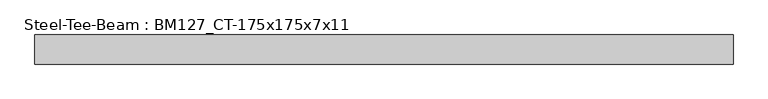
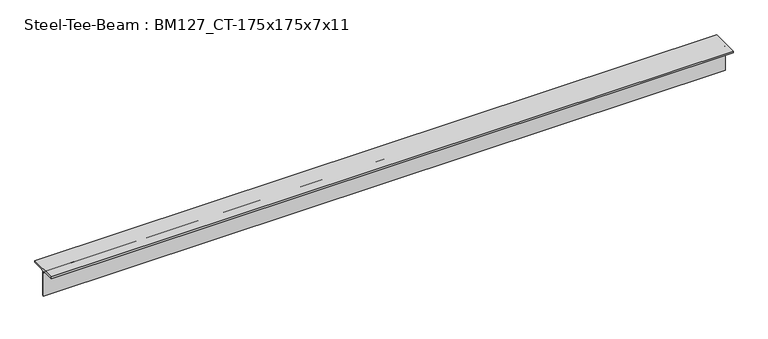
"""IFC4 building model written with IfcOpenShell, lengths in millimetres: beam geometry, Steel-Tee-Beam : BM127_CT-175x175x7x11."""

import ifcopenshell
import ifcopenshell.guid

model = None  # the IFC model being written
_history = None  # IfcOwnerHistory: only IFC2X3 demands one
_inside = {}  # id of a spatial element -> (the spatial element, [elements in it])
_under = {}  # id of a project, library or spatial element -> (it, [spatial elements below it])
_declared = {}  # id of a project -> (the project, [libraries it declares])
_typed = {}  # id of a type object -> (the type object, [elements of that type])
_made_of = {}  # id of a material, layer set ... -> (it, [elements and type objects made of it])


def new_model(schema):
    """Start an empty IFC model of exactly this schema.

    Asked for "IFC4X3", IfcOpenShell would pick the latest addendum, in which some entities
    have other attributes; the version numbers below select the first issue.
    IFC2X3 requires an IfcOwnerHistory on every rooted entity: one is made here for all.
    """
    global model, _history
    if schema == "IFC4X3":
        model = ifcopenshell.file(schema_version=(4, 3, 0, 0))
    else:
        model = ifcopenshell.file(schema=schema)
    _inside.clear()
    _under.clear()
    _declared.clear()
    _typed.clear()
    _made_of.clear()
    _history = None
    if model.schema == "IFC2X3":
        org = make("IfcOrganization", Name="unknown")
        user = make(
            "IfcPersonAndOrganization",
            ThePerson=make("IfcPerson", FamilyName="unknown"),
            TheOrganization=org,
        )
        app = make(
            "IfcApplication",
            ApplicationDeveloper=org,
            Version="unknown",
            ApplicationFullName="unknown",
            ApplicationIdentifier="unknown",
        )
        _history = make(
            "IfcOwnerHistory",
            OwningUser=user,
            OwningApplication=app,
            ChangeAction="ADDED",
            CreationDate=0,
        )
    return model


def make(cls, **values):
    """One entity of the class cls with the attributes given. An attribute that is None is left unset."""
    return model.create_entity(
        cls, **{name: value for name, value in values.items() if value is not None}
    )


def rooted(cls, **values):
    """An entity with a GlobalId (a new one), such as an element, a storey or a relation."""
    return make(cls, GlobalId=ifcopenshell.guid.new(), OwnerHistory=_history, **values)


def si_unit(unit_type, name, prefix=None):
    """IfcSIUnit, for example si_unit("LENGTHUNIT", "METRE", prefix="MILLI")."""
    return make("IfcSIUnit", UnitType=unit_type, Prefix=prefix, Name=name)


def assignment(units):
    """IfcUnitAssignment: the units of a project."""
    return None if units is None else make("IfcUnitAssignment", Units=units)


def point(xyz):
    """IfcCartesianPoint."""
    return None if xyz is None else make("IfcCartesianPoint", Coordinates=xyz)


def direction(xyz):
    """IfcDirection."""
    return None if xyz is None else make("IfcDirection", DirectionRatios=xyz)


def frame(location, z_axis=None, x_axis=None):
    """IfcAxis2Placement3D, a coordinate frame: its origin and axes. An axis left out is left unset."""
    return make(
        "IfcAxis2Placement3D",
        Location=point(location),
        Axis=direction(z_axis),
        RefDirection=direction(x_axis),
    )


def frame_2d(location, x_axis=None):
    """IfcAxis2Placement2D, a coordinate frame in the plane: its origin and x axis."""
    return make(
        "IfcAxis2Placement2D", Location=point(location), RefDirection=direction(x_axis)
    )


def origin():
    """The frame at (0, 0, 0) with its axes left unset."""
    return frame((0.0, 0.0, 0.0))


def place(relative_to, where):
    """IfcLocalPlacement: puts the frame where relative to a parent placement (None: the world)."""
    return make(
        "IfcLocalPlacement", PlacementRelTo=relative_to, RelativePlacement=where
    )


def context(
    kind, dimensions, precision=None, world=None, true_north=None, identifier=None
):
    """IfcGeometricRepresentationContext, for example the 3D "Model" context."""
    return make(
        "IfcGeometricRepresentationContext",
        ContextIdentifier=identifier,
        ContextType=kind,
        CoordinateSpaceDimension=dimensions,
        Precision=precision,
        WorldCoordinateSystem=world,
        TrueNorth=true_north,
    )


def project(units=None, contexts=None):
    """IfcProject with its units and contexts."""
    return rooted(
        "IfcProject",
        Name="project",
        RepresentationContexts=contexts,
        UnitsInContext=assignment(units),
    )


def spatial(cls, under=None, at=None, **own):
    """A site, building, storey or space (cls), placed at a placement, below another one or the project."""
    s = rooted(cls, ObjectPlacement=at, **own)
    if under is not None:
        _under.setdefault(under.id(), (under, []))[1].append(s)
    return s


def polyline(points):
    """IfcPolyline through the points."""
    return make("IfcPolyline", Points=[point(p) for p in points])


def circle_curve(where, radius):
    """IfcCircle in the frame where."""
    return make("IfcCircle", Position=where, Radius=radius)


def trimmed(basis, trim1, trim2, sense, master):
    """IfcTrimmedCurve: the piece of a basis curve between two trims."""
    return make(
        "IfcTrimmedCurve",
        BasisCurve=basis,
        Trim1=trim1,
        Trim2=trim2,
        SenseAgreement=sense,
        MasterRepresentation=master,
    )


def segment(curve, same_sense, transition):
    """IfcCompositeCurveSegment."""
    return make(
        "IfcCompositeCurveSegment",
        Transition=transition,
        SameSense=same_sense,
        ParentCurve=curve,
    )


def composite_curve(segments, self_intersect=None):
    """IfcCompositeCurve: segments joined end to end."""
    return make("IfcCompositeCurve", Segments=segments, SelfIntersect=self_intersect)


def outline(outer, holes=None, kind="AREA"):
    """IfcArbitraryClosedProfileDef: a profile drawn as a closed curve; with holes, ...WithVoids."""
    if holes is None:
        return make("IfcArbitraryClosedProfileDef", ProfileType=kind, OuterCurve=outer)
    return make(
        "IfcArbitraryProfileDefWithVoids",
        ProfileType=kind,
        OuterCurve=outer,
        InnerCurves=holes,
    )


def extrude(swept, where, along, depth):
    """IfcExtrudedAreaSolid: the profile swept, set in the frame where, extruded along a direction by depth."""
    return make(
        "IfcExtrudedAreaSolid",
        SweptArea=swept,
        Position=where,
        ExtrudedDirection=direction(along),
        Depth=depth,
    )


def shape(context_of_items, identifier, shape_type, items):
    """IfcShapeRepresentation: the items that make up one representation, for example the "Body"."""
    return make(
        "IfcShapeRepresentation",
        ContextOfItems=context_of_items,
        RepresentationIdentifier=identifier,
        RepresentationType=shape_type,
        Items=items,
    )


def source(mapping_origin, context_of_items, identifier, shape_type, items):
    """IfcRepresentationMap: a shape defined once, which mapped items show again and again."""
    return make(
        "IfcRepresentationMap",
        MappingOrigin=mapping_origin,
        MappedRepresentation=shape(context_of_items, identifier, shape_type, items),
    )


def transform(
    local_origin,
    x_axis=None,
    y_axis=None,
    z_axis=None,
    scale=None,
    scale2=None,
    scale3=None,
    uniform=True,
):
    """IfcCartesianTransformationOperator3D, or its non-uniform kind. x_axis, y_axis, z_axis: its Axis1, 2, 3."""
    if uniform:
        return make(
            "IfcCartesianTransformationOperator3D",
            Axis1=direction(x_axis),
            Axis2=direction(y_axis),
            LocalOrigin=point(local_origin),
            Scale=scale,
            Axis3=direction(z_axis),
        )
    return make(
        "IfcCartesianTransformationOperator3DnonUniform",
        Axis1=direction(x_axis),
        Axis2=direction(y_axis),
        LocalOrigin=point(local_origin),
        Scale=scale,
        Axis3=direction(z_axis),
        Scale2=scale2,
        Scale3=scale3,
    )


def mapped(mapping_source, mapping_target):
    """IfcMappedItem: shows the shape of a source again, moved by a transform."""
    return make(
        "IfcMappedItem", MappingSource=mapping_source, MappingTarget=mapping_target
    )


def made_of(thing, what):
    """Note that an element or type object is made of a material, layer set ...; save() writes the relation."""
    if what is not None:
        _made_of.setdefault(what.id(), (what, []))[1].append(thing)
    return thing


def element(
    cls,
    number,
    at=None,
    inside=None,
    cuts=None,
    type_object=None,
    material=None,
    context=None,
    identifier="Body",
    shape_type=None,
    held_by="IfcProductDefinitionShape",
    body=None,
    shapes=None,
    **own,
):
    """One element of the class cls, such as IfcWall. Its Tag is "e" and its number.

    at: its placement. inside: the storey or other place that contains it. cuts: it is an
    opening in that element (IfcRelVoidsElement). A single representation is given by context,
    identifier, shape_type and body (its items); several are given by shapes. held_by: the class
    of the entity that holds the representations. save() writes the other relations.
    """
    e = rooted(cls, Tag="e%d" % number, ObjectPlacement=at, **own)
    if body is not None:
        shapes = [shape(context, identifier, shape_type, body)]
    if shapes is not None:
        e.Representation = make(held_by, Representations=shapes)
    if inside is not None:
        _inside.setdefault(inside.id(), (inside, []))[1].append(e)
    if cuts is not None:
        rooted(
            "IfcRelVoidsElement", RelatingBuildingElement=cuts, RelatedOpeningElement=e
        )
    if type_object is not None:
        _typed.setdefault(type_object.id(), (type_object, []))[1].append(e)
    return made_of(e, material)


def aggregate(whole, parts):
    """IfcRelAggregates: a whole, such as a stair, and the parts it consists of."""
    return rooted("IfcRelAggregates", RelatingObject=whole, RelatedObjects=parts)


def save(model, path):
    """Write the relations noted so far, then the file.

    IfcRelAggregates (storeys below a building ...), IfcRelContainedInSpatialStructure (elements
    in a storey), IfcRelDefinesByType, IfcRelAssociatesMaterial and IfcRelDeclares: one each for
    every whole, place, type object, material and project.
    """
    for whole, parts in _under.values():
        aggregate(whole, parts)
    for where, things in _inside.values():
        rooted(
            "IfcRelContainedInSpatialStructure",
            RelatedElements=things,
            RelatingStructure=where,
        )
    for kind, things in _typed.values():
        rooted("IfcRelDefinesByType", RelatedObjects=things, RelatingType=kind)
    for what, things in _made_of.values():
        rooted("IfcRelAssociatesMaterial", RelatedObjects=things, RelatingMaterial=what)
    for by, libraries in _declared.values():
        rooted("IfcRelDeclares", RelatingContext=by, RelatedDefinitions=libraries)
    model.write(path)


def steel_tee_beam_bm127_ct_175x175x7x11_36c48f08(model_context):
    return source(origin(), model_context, "Body", "SweptSolid", [
        extrude(outline(composite_curve([segment(polyline([(87.5, 87.5), (87.5, 76.5), (17.5, 76.5)]), True, "CONTINUOUS"), segment(trimmed(circle_curve(frame_2d((17.5, 62.5)), 14.0), [point((17.5, 76.5))], [point((3.5, 62.5))], True, "CARTESIAN"), True, "CONTINUOUS"), segment(polyline([(3.5, 62.5), (3.5, -87.5), (-3.5, -87.5), (-3.5, 62.5)]), True, "CONTINUOUS"), segment(trimmed(circle_curve(frame_2d((-17.5, 62.5)), 14.0), [point((-3.5, 62.5))], [point((-17.5, 76.5))], True, "CARTESIAN"), True, "CONTINUOUS"), segment(polyline([(-17.5, 76.5), (-87.5, 76.5), (-87.5, 87.5), (87.5, 87.5)]), True, "CONTINUOUS")], self_intersect=False)), frame((-1998.4928423, 0.0, 0.0), z_axis=(1.0, 0.0, 0.0), x_axis=(0.0, 1.0, 0.0)), (0.0, 0.0, 1.0), 4194.118334),
    ])


if __name__ == "__main__":
    model = new_model("IFC4")
    model_context = context("Model", 3, world=origin())
    ifc_project = project(units=[si_unit("LENGTHUNIT", "METRE", prefix="MILLI")], contexts=[model_context])
    site = spatial("IfcSite", under=ifc_project)
    building = spatial("IfcBuilding", under=site)
    placement = place(None, origin())
    steel_tee_beam_bm127_ct_175x175x7x11_shape = steel_tee_beam_bm127_ct_175x175x7x11_36c48f08(model_context)
    element("IfcBeam", 1, ObjectType="Steel-Tee-Beam : BM127_CT-175x175x7x11", at=placement, inside=building, context=model_context, shape_type="MappedRepresentation", body=[
        mapped(steel_tee_beam_bm127_ct_175x175x7x11_shape, transform((0.0, 0.0, 0.0), x_axis=(1.0, 0.0, 0.0), y_axis=(0.0, 1.0, 0.0), z_axis=(0.0, 0.0, 1.0))),
    ])
    save(model, "model.ifc")

# Revit data of these elements
# Type "Steel-Tee-Beam : BM127_CT-175x175x7x11"
#   Surface Area = 0.687982 m²/m
#   Section Area = 31.5712 cm²
#   Mass per Unit Length = 24.7834 kg/m
#   Length [instance default] = 1524 mm
#   bf = 175 mm
#   d = 175 mm
#   k = 25 mm
#   r = 14 mm
#   tf = 11 mm
#   tw = 7 mm
#   hec_material4 [instance default] = none
#   hec_material3 [instance default] = none
#   hec_material2 [instance default] = none
#   hec_material1 [instance default] = none
#   Structural Material [instance default] = Steel, 45-345
#   Assembly Code = ""
# Element 1 (IfcBeam, "Steel-Tee-Beam : BM127_CT-175x175x7x11")
#   hec_material3 = F01AC000-00002_Building/Shelter Fire Proofing Work_Intumescent Coating Type_1 hr. rating (UL 1709))
#   hec_material2 = S01AA010-00002_Main Steel Structure Fabrication Work_Shelter/Building_Steel Painting/Coating_for Fireproofed Steel Surface, Surface Preparation & Primer Coat
#   hec_material1 = S03AA029-00001_Main Steel Structure Erection Work_Shelter/Building_Light Steel
#   Structural Material = S01AA003-00001_Main Steel Structure Fabrication Work_Shelter/Building_Light Steel - Standard
#   Materials on its faces: "S01AA003-00001_Main Steel Structure Fabrication Work_Shelter/Building_Light Steel - Standard"
# Materials
#   "Steel, 45-345": class "Metal", colour RGB 189 187 185, transparency 0, Description = "Steel 345 MPa", Cost = 0
#   "S01AA003-00001_Main Steel Structure Fabrication Work_Shelter/Building_Light Steel - Standard": class "Metal", colour RGB 120 120 120, transparency 0, Comments = "(30KG/M>Weight)", Description = "Structural steel 50ksi", W00) Work Master Code = "S01AA003-00001", W01) Work Master_Lv1 = "Main Steel Structure Fabrication Work", W02) Work Master_Lv2 = "Shelter/Building", W03) Work Master_Spec.1 = "Light Steel - Standard (30KG/M>Weight)", Cost = 0
#   "F01AC000-00002_Building/Shelter Fire Proofing Work_Intumescent Coating Type_1 hr. rating (UL 1709))": class "Metal", colour RGB 255 128 128, transparency 0, Description = "Paint finished steel", W00) Work Master Code = "F01AC000-00002", W01) Work Master_Lv1 = "Building/Shelter Fire Proofing Work", W02) Work Master_Lv2 = "Intumescent Coating Type", W03) Work Master_Spec.1 = "1 hr. rating (UL 1709)", Cost = 0
#   "S01AA010-00002_Main Steel Structure Fabrication Work_Shelter/Building_Steel Painting/Coating_for Fireproofed Steel Surface, Surface Preparation & Primer Coat": class "Metal", colour RGB 120 120 120, transparency 0, Description = "Paint finished steel", W00) Work Master Code = "SS01AA010-00002", W01) Work Master_Lv1 = "Main Steel Structure Fabrication Work", W02) Work Master_Lv2 = "Shelter/Building", W03) Work Master_Spec.1 = "Steel Painting/Coating", W04) Work Master_Spec.2 = "for Fireproofed Steel Surface, Surface Preparation & Primer Coat", Cost = 0
#   "S03AA029-00001_Main Steel Structure Erection Work_Shelter/Building_Light Steel": class "Metal", colour RGB 120 120 120, transparency 0, Comments = "(30KG/M>Weight)", Description = "Structural steel 50ksi", W00) Work Master Code = "S03AA029-00001", W01) Work Master_Lv1 = "Main Steel Structure Erection Work", W02) Work Master_Lv2 = "Shelter/Building", W03) Work Master_Spec.1 = "Light Steel (30KG/M>Weight)", Cost = 0
